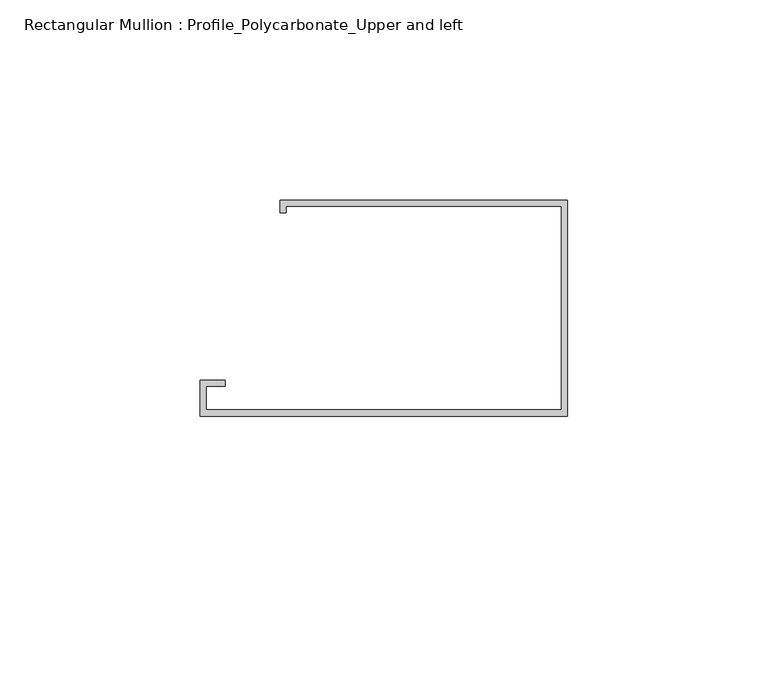
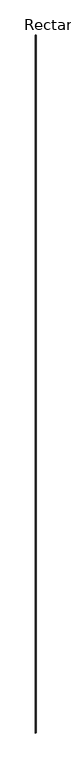
"""IFC4 building model written with IfcOpenShell, lengths in millimetres: member geometry, Rectangular Mullion : Profile_Polycarbonate_Upper and left."""

from ifc_helpers import new_model, si_unit, frame, origin, place, context, project, spatial, polyline, outline, extrude, source, transform, mapped, element, save


def rectangular_mullion_profile_polycarbonate_upper_and_left_5d9afb4b(model_context):
    return source(origin(), model_context, "Body", "SweptSolid", [
        extrude(outline(polyline([(0.0, -28.984575), (-91.9988, -28.984575), (-91.9988, -19.992975), (-85.6488, -19.992975), (-85.6488, -21.580475), (-90.4113, -21.580475), (-90.4113, -27.397075), (-1.5875, -27.397075), (-1.5875, 23.428325), (-70.3961, 23.428325), (-70.3961, 21.840825), (-71.9836, 21.840825), (-71.9836, 25.015825), (0.0, 25.015825), (0.0, -28.984575)])), frame((0.0, 0.0, -81115.1885281), z_axis=(0.0, 0.0, 1.0), x_axis=(1.0, 0.0, 0.0)), (0.0, 0.0, 1.0), 81115.1885281),
    ])


if __name__ == "__main__":
    model = new_model("IFC4")
    model_context = context("Model", 3, world=origin())
    ifc_project = project(units=[si_unit("LENGTHUNIT", "METRE", prefix="MILLI")], contexts=[model_context])
    site = spatial("IfcSite", under=ifc_project)
    building = spatial("IfcBuilding", under=site)
    placement = place(None, origin())
    rectangular_mullion_profile_polycarbonate_upper_and_left_shape = rectangular_mullion_profile_polycarbonate_upper_and_left_5d9afb4b(model_context)
    element("IfcMember", 1, ObjectType="Rectangular Mullion : Profile_Polycarbonate_Upper and left", at=placement, inside=building, context=model_context, shape_type="MappedRepresentation", body=[
        mapped(rectangular_mullion_profile_polycarbonate_upper_and_left_shape, transform((0.0, 0.0, 0.0), x_axis=(1.0, 0.0, 0.0), y_axis=(0.0, 1.0, 0.0), z_axis=(0.0, 0.0, 1.0))),
    ])
    save(model, "model.ifc")

# Revit data of these elements
# Type "Rectangular Mullion : Profile_Polycarbonate_Upper and left"
#   built-in parameter 1007322 = 0.177167 (stored number, unit not read)
#   built-in parameter 1007321 = 0.00520833 (stored number, unit not read)
#   built-in parameter 1007320 = 0 (stored number, unit not read)
